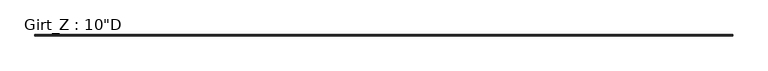
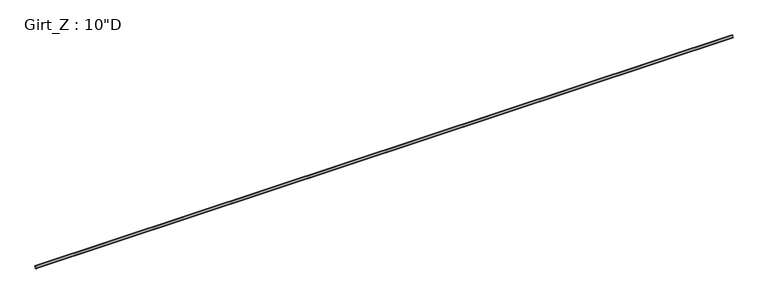
"""IFC4 building model written with IfcOpenShell, lengths in millimetres: beam geometry."""

from ifc_helpers import new_model, si_unit, point, frame, frame_2d, origin, place, context, project, spatial, polyline, circle_curve, trimmed, segment, composite_curve, outline, extrude, source, transform, mapped, element, save


def beam_abf8bc6d(model_context):
    return source(origin(), model_context, "Body", "SweptSolid", [
        extrude(outline(composite_curve([segment(polyline([(63.5, 127.0), (75.745104, 112.4068534), (73.6169367, 110.621109), (62.204539, 124.221875), (3.3005807, 124.221875)]), True, "CONTINUOUS"), segment(trimmed(circle_curve(frame_2d((3.3741066, 122.2381931)), 1.9850441), [point((3.3005807, 124.221875))], [point((1.3890625, 122.2381931))], True, "CARTESIAN"), True, "CONTINUOUS"), segment(polyline([(1.3890625, 122.2381931), (1.3890625, -122.2375)]), True, "CONTINUOUS"), segment(trimmed(circle_curve(frame_2d((-3.3734375, -122.2375)), 4.7625), [point((1.3890625, -122.2375))], [point((-3.3734375, -127.0))], False, "CARTESIAN"), True, "CONTINUOUS"), segment(polyline([(-3.3734375, -127.0), (-63.5, -127.0), (-75.745104, -112.4068534), (-73.6169367, -110.621109), (-62.204539, -124.221875), (-3.2694106, -124.221875)]), True, "CONTINUOUS"), segment(trimmed(circle_curve(frame_2d((-3.3748024, -122.2389339)), 1.9857399), [point((-3.2694106, -124.221875))], [point((-1.3890625, -122.2389339))], True, "CARTESIAN"), True, "CONTINUOUS"), segment(polyline([(-1.3890625, -122.2389339), (-1.3890625, 122.2375)]), True, "CONTINUOUS"), segment(trimmed(circle_curve(frame_2d((3.3734375, 122.2375)), 4.7625), [point((-1.3890625, 122.2375))], [point((3.3734375, 127.0))], False, "CARTESIAN"), True, "CONTINUOUS"), segment(polyline([(3.3734375, 127.0), (63.5, 127.0)]), True, "CONTINUOUS")], self_intersect=False)), frame((-40373.3, 0.0, 0.0), z_axis=(1.0, 0.0, 0.0), x_axis=(0.0, 1.0, 0.0)), (0.0, 0.0, 1.0), 80505.3),
    ])


if __name__ == "__main__":
    model = new_model("IFC4")
    model_context = context("Model", 3, world=origin())
    ifc_project = project(units=[si_unit("LENGTHUNIT", "METRE", prefix="MILLI")], contexts=[model_context])
    site = spatial("IfcSite", under=ifc_project)
    building = spatial("IfcBuilding", under=site)
    placement = place(None, origin())
    beam_shape = beam_abf8bc6d(model_context)
    element("IfcBeam", 1, ObjectType="Girt_Z : 10\"D", at=placement, inside=building, context=model_context, shape_type="MappedRepresentation", body=[
        mapped(beam_shape, transform((0.0, 0.0, 0.0), x_axis=(1.0, 0.0, 0.0), y_axis=(0.0, 1.0, 0.0), z_axis=(0.0, 0.0, 1.0))),
    ])
    save(model, "model.ifc")

# Revit data of these elements
# Type "Girt_Z : 10\"D"
#   Web_Thickness = 0' - 0 7/64"
#   Length [instance default] = 10' - 0"
#   Leg_1 = 0' - 2 1/2"
#   Height = 0' - 10"
#   Structural Material [instance default] = none
